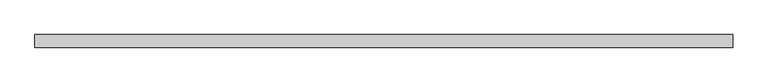
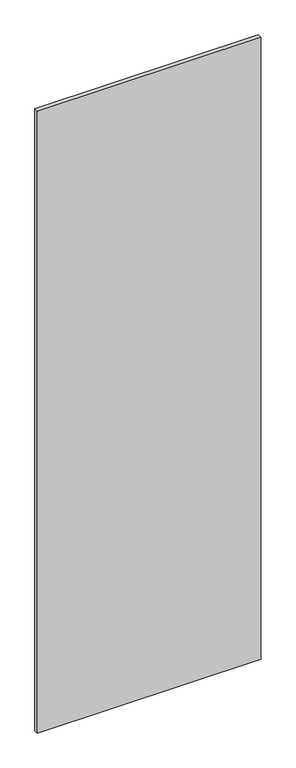
"""IFC4 building model written with IfcOpenShell, lengths in millimetres: plate geometry, 系统嵌板 : 玻璃."""

import ifcopenshell
import ifcopenshell.guid

model = None  # the IFC model being written
_history = None  # IfcOwnerHistory: only IFC2X3 demands one
_inside = {}  # id of a spatial element -> (the spatial element, [elements in it])
_under = {}  # id of a project, library or spatial element -> (it, [spatial elements below it])
_declared = {}  # id of a project -> (the project, [libraries it declares])
_typed = {}  # id of a type object -> (the type object, [elements of that type])
_made_of = {}  # id of a material, layer set ... -> (it, [elements and type objects made of it])


def new_model(schema):
    """Start an empty IFC model of exactly this schema.

    Asked for "IFC4X3", IfcOpenShell would pick the latest addendum, in which some entities
    have other attributes; the version numbers below select the first issue.
    IFC2X3 requires an IfcOwnerHistory on every rooted entity: one is made here for all.
    """
    global model, _history
    if schema == "IFC4X3":
        model = ifcopenshell.file(schema_version=(4, 3, 0, 0))
    else:
        model = ifcopenshell.file(schema=schema)
    _inside.clear()
    _under.clear()
    _declared.clear()
    _typed.clear()
    _made_of.clear()
    _history = None
    if model.schema == "IFC2X3":
        org = make("IfcOrganization", Name="unknown")
        user = make(
            "IfcPersonAndOrganization",
            ThePerson=make("IfcPerson", FamilyName="unknown"),
            TheOrganization=org,
        )
        app = make(
            "IfcApplication",
            ApplicationDeveloper=org,
            Version="unknown",
            ApplicationFullName="unknown",
            ApplicationIdentifier="unknown",
        )
        _history = make(
            "IfcOwnerHistory",
            OwningUser=user,
            OwningApplication=app,
            ChangeAction="ADDED",
            CreationDate=0,
        )
    return model


def make(cls, **values):
    """One entity of the class cls with the attributes given. An attribute that is None is left unset."""
    return model.create_entity(
        cls, **{name: value for name, value in values.items() if value is not None}
    )


def rooted(cls, **values):
    """An entity with a GlobalId (a new one), such as an element, a storey or a relation."""
    return make(cls, GlobalId=ifcopenshell.guid.new(), OwnerHistory=_history, **values)


def si_unit(unit_type, name, prefix=None):
    """IfcSIUnit, for example si_unit("LENGTHUNIT", "METRE", prefix="MILLI")."""
    return make("IfcSIUnit", UnitType=unit_type, Prefix=prefix, Name=name)


def assignment(units):
    """IfcUnitAssignment: the units of a project."""
    return None if units is None else make("IfcUnitAssignment", Units=units)


def point(xyz):
    """IfcCartesianPoint."""
    return None if xyz is None else make("IfcCartesianPoint", Coordinates=xyz)


def direction(xyz):
    """IfcDirection."""
    return None if xyz is None else make("IfcDirection", DirectionRatios=xyz)


def frame(location, z_axis=None, x_axis=None):
    """IfcAxis2Placement3D, a coordinate frame: its origin and axes. An axis left out is left unset."""
    return make(
        "IfcAxis2Placement3D",
        Location=point(location),
        Axis=direction(z_axis),
        RefDirection=direction(x_axis),
    )


def origin():
    """The frame at (0, 0, 0) with its axes left unset."""
    return frame((0.0, 0.0, 0.0))


def origin_with_axes():
    """The frame at (0, 0, 0) with the z axis (0, 0, 1) and the x axis (1, 0, 0) written out."""
    return frame((0.0, 0.0, 0.0), z_axis=(0.0, 0.0, 1.0), x_axis=(1.0, 0.0, 0.0))


def place(relative_to, where):
    """IfcLocalPlacement: puts the frame where relative to a parent placement (None: the world)."""
    return make(
        "IfcLocalPlacement", PlacementRelTo=relative_to, RelativePlacement=where
    )


def context(
    kind, dimensions, precision=None, world=None, true_north=None, identifier=None
):
    """IfcGeometricRepresentationContext, for example the 3D "Model" context."""
    return make(
        "IfcGeometricRepresentationContext",
        ContextIdentifier=identifier,
        ContextType=kind,
        CoordinateSpaceDimension=dimensions,
        Precision=precision,
        WorldCoordinateSystem=world,
        TrueNorth=true_north,
    )


def project(units=None, contexts=None):
    """IfcProject with its units and contexts."""
    return rooted(
        "IfcProject",
        Name="project",
        RepresentationContexts=contexts,
        UnitsInContext=assignment(units),
    )


def spatial(cls, under=None, at=None, **own):
    """A site, building, storey or space (cls), placed at a placement, below another one or the project."""
    s = rooted(cls, ObjectPlacement=at, **own)
    if under is not None:
        _under.setdefault(under.id(), (under, []))[1].append(s)
    return s


def polyline(points):
    """IfcPolyline through the points."""
    return make("IfcPolyline", Points=[point(p) for p in points])


def outline(outer, holes=None, kind="AREA"):
    """IfcArbitraryClosedProfileDef: a profile drawn as a closed curve; with holes, ...WithVoids."""
    if holes is None:
        return make("IfcArbitraryClosedProfileDef", ProfileType=kind, OuterCurve=outer)
    return make(
        "IfcArbitraryProfileDefWithVoids",
        ProfileType=kind,
        OuterCurve=outer,
        InnerCurves=holes,
    )


def extrude(swept, where, along, depth):
    """IfcExtrudedAreaSolid: the profile swept, set in the frame where, extruded along a direction by depth."""
    return make(
        "IfcExtrudedAreaSolid",
        SweptArea=swept,
        Position=where,
        ExtrudedDirection=direction(along),
        Depth=depth,
    )


def shape(context_of_items, identifier, shape_type, items):
    """IfcShapeRepresentation: the items that make up one representation, for example the "Body"."""
    return make(
        "IfcShapeRepresentation",
        ContextOfItems=context_of_items,
        RepresentationIdentifier=identifier,
        RepresentationType=shape_type,
        Items=items,
    )


def source(mapping_origin, context_of_items, identifier, shape_type, items):
    """IfcRepresentationMap: a shape defined once, which mapped items show again and again."""
    return make(
        "IfcRepresentationMap",
        MappingOrigin=mapping_origin,
        MappedRepresentation=shape(context_of_items, identifier, shape_type, items),
    )


def transform(
    local_origin,
    x_axis=None,
    y_axis=None,
    z_axis=None,
    scale=None,
    scale2=None,
    scale3=None,
    uniform=True,
):
    """IfcCartesianTransformationOperator3D, or its non-uniform kind. x_axis, y_axis, z_axis: its Axis1, 2, 3."""
    if uniform:
        return make(
            "IfcCartesianTransformationOperator3D",
            Axis1=direction(x_axis),
            Axis2=direction(y_axis),
            LocalOrigin=point(local_origin),
            Scale=scale,
            Axis3=direction(z_axis),
        )
    return make(
        "IfcCartesianTransformationOperator3DnonUniform",
        Axis1=direction(x_axis),
        Axis2=direction(y_axis),
        LocalOrigin=point(local_origin),
        Scale=scale,
        Axis3=direction(z_axis),
        Scale2=scale2,
        Scale3=scale3,
    )


def mapped(mapping_source, mapping_target):
    """IfcMappedItem: shows the shape of a source again, moved by a transform."""
    return make(
        "IfcMappedItem", MappingSource=mapping_source, MappingTarget=mapping_target
    )


def made_of(thing, what):
    """Note that an element or type object is made of a material, layer set ...; save() writes the relation."""
    if what is not None:
        _made_of.setdefault(what.id(), (what, []))[1].append(thing)
    return thing


def element(
    cls,
    number,
    at=None,
    inside=None,
    cuts=None,
    type_object=None,
    material=None,
    context=None,
    identifier="Body",
    shape_type=None,
    held_by="IfcProductDefinitionShape",
    body=None,
    shapes=None,
    **own,
):
    """One element of the class cls, such as IfcWall. Its Tag is "e" and its number.

    at: its placement. inside: the storey or other place that contains it. cuts: it is an
    opening in that element (IfcRelVoidsElement). A single representation is given by context,
    identifier, shape_type and body (its items); several are given by shapes. held_by: the class
    of the entity that holds the representations. save() writes the other relations.
    """
    e = rooted(cls, Tag="e%d" % number, ObjectPlacement=at, **own)
    if body is not None:
        shapes = [shape(context, identifier, shape_type, body)]
    if shapes is not None:
        e.Representation = make(held_by, Representations=shapes)
    if inside is not None:
        _inside.setdefault(inside.id(), (inside, []))[1].append(e)
    if cuts is not None:
        rooted(
            "IfcRelVoidsElement", RelatingBuildingElement=cuts, RelatedOpeningElement=e
        )
    if type_object is not None:
        _typed.setdefault(type_object.id(), (type_object, []))[1].append(e)
    return made_of(e, material)


def aggregate(whole, parts):
    """IfcRelAggregates: a whole, such as a stair, and the parts it consists of."""
    return rooted("IfcRelAggregates", RelatingObject=whole, RelatedObjects=parts)


def save(model, path):
    """Write the relations noted so far, then the file.

    IfcRelAggregates (storeys below a building ...), IfcRelContainedInSpatialStructure (elements
    in a storey), IfcRelDefinesByType, IfcRelAssociatesMaterial and IfcRelDeclares: one each for
    every whole, place, type object, material and project.
    """
    for whole, parts in _under.values():
        aggregate(whole, parts)
    for where, things in _inside.values():
        rooted(
            "IfcRelContainedInSpatialStructure",
            RelatedElements=things,
            RelatingStructure=where,
        )
    for kind, things in _typed.values():
        rooted("IfcRelDefinesByType", RelatedObjects=things, RelatingType=kind)
    for what, things in _made_of.values():
        rooted("IfcRelAssociatesMaterial", RelatedObjects=things, RelatingMaterial=what)
    for by, libraries in _declared.values():
        rooted("IfcRelDeclares", RelatingContext=by, RelatedDefinitions=libraries)
    model.write(path)


def plate_e4d7b700(model_context):
    return source(origin(), model_context, "Body", "SweptSolid", [
        extrude(outline(polyline([(680.0, -12.5), (-680.0, -12.5), (-680.0, 12.5), (680.0, 12.5), (680.0, -12.5)])), origin_with_axes(), (0.0, 0.0, 1.0), 4000.0),
    ])


if __name__ == "__main__":
    model = new_model("IFC4")
    model_context = context("Model", 3, world=origin())
    ifc_project = project(units=[si_unit("LENGTHUNIT", "METRE", prefix="MILLI")], contexts=[model_context])
    site = spatial("IfcSite", under=ifc_project)
    building = spatial("IfcBuilding", under=site)
    placement = place(None, origin())
    plate_shape = plate_e4d7b700(model_context)
    element("IfcPlate", 1, ObjectType="系统嵌板 : 玻璃", at=placement, inside=building, context=model_context, shape_type="MappedRepresentation", body=[
        mapped(plate_shape, transform((0.0, 0.0, 0.0), x_axis=(1.0, 0.0, 0.0), y_axis=(0.0, 1.0, 0.0), z_axis=(0.0, 0.0, 1.0))),
    ])
    save(model, "model.ifc")

# Revit data of these elements
# Type "系统嵌板 : 玻璃"
#   Construction Type Id = "GSP4R"
#   Analytic Construction = "1/8 英寸 Pilkington 单层玻璃"
#   Visual Light Transmittance = 0.9
#   Solar Heat Gain Coefficient = 0.86
#   Heat Transfer Coefficient (U) = 6.7069 W/(m²·K)
# Element 1 (IfcPlate, "系统嵌板 : 玻璃")
#   Materials on its faces: "玻璃"
# Materials
#   "玻璃": class "玻璃", colour RGB 0 128 192, transparency 0.9, Description = "钠钙玻璃", Cost = 0
